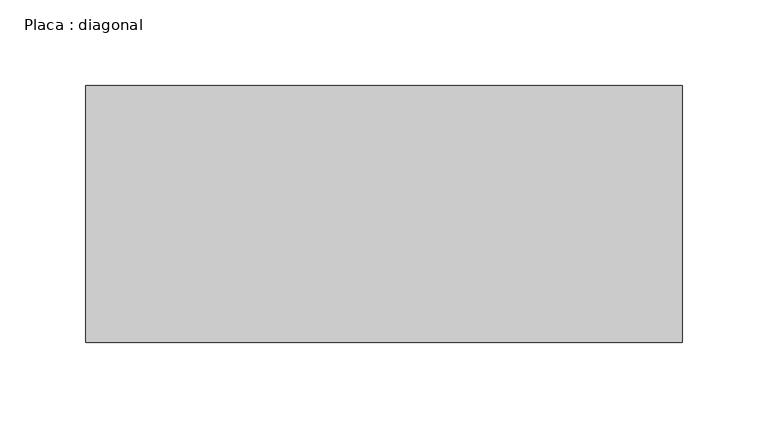
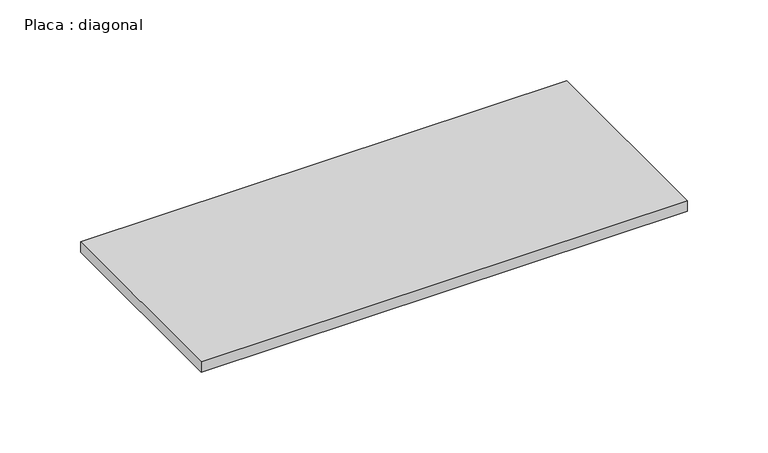
"""IFC4 building model written with IfcOpenShell, lengths in millimetres: beam geometry, Placa : diagonal."""

import ifcopenshell
import ifcopenshell.guid

model = None  # the IFC model being written
_history = None  # IfcOwnerHistory: only IFC2X3 demands one
_inside = {}  # id of a spatial element -> (the spatial element, [elements in it])
_under = {}  # id of a project, library or spatial element -> (it, [spatial elements below it])
_declared = {}  # id of a project -> (the project, [libraries it declares])
_typed = {}  # id of a type object -> (the type object, [elements of that type])
_made_of = {}  # id of a material, layer set ... -> (it, [elements and type objects made of it])


def new_model(schema):
    """Start an empty IFC model of exactly this schema.

    Asked for "IFC4X3", IfcOpenShell would pick the latest addendum, in which some entities
    have other attributes; the version numbers below select the first issue.
    IFC2X3 requires an IfcOwnerHistory on every rooted entity: one is made here for all.
    """
    global model, _history
    if schema == "IFC4X3":
        model = ifcopenshell.file(schema_version=(4, 3, 0, 0))
    else:
        model = ifcopenshell.file(schema=schema)
    _inside.clear()
    _under.clear()
    _declared.clear()
    _typed.clear()
    _made_of.clear()
    _history = None
    if model.schema == "IFC2X3":
        org = make("IfcOrganization", Name="unknown")
        user = make(
            "IfcPersonAndOrganization",
            ThePerson=make("IfcPerson", FamilyName="unknown"),
            TheOrganization=org,
        )
        app = make(
            "IfcApplication",
            ApplicationDeveloper=org,
            Version="unknown",
            ApplicationFullName="unknown",
            ApplicationIdentifier="unknown",
        )
        _history = make(
            "IfcOwnerHistory",
            OwningUser=user,
            OwningApplication=app,
            ChangeAction="ADDED",
            CreationDate=0,
        )
    return model


def make(cls, **values):
    """One entity of the class cls with the attributes given. An attribute that is None is left unset."""
    return model.create_entity(
        cls, **{name: value for name, value in values.items() if value is not None}
    )


def rooted(cls, **values):
    """An entity with a GlobalId (a new one), such as an element, a storey or a relation."""
    return make(cls, GlobalId=ifcopenshell.guid.new(), OwnerHistory=_history, **values)


def si_unit(unit_type, name, prefix=None):
    """IfcSIUnit, for example si_unit("LENGTHUNIT", "METRE", prefix="MILLI")."""
    return make("IfcSIUnit", UnitType=unit_type, Prefix=prefix, Name=name)


def assignment(units):
    """IfcUnitAssignment: the units of a project."""
    return None if units is None else make("IfcUnitAssignment", Units=units)


def point(xyz):
    """IfcCartesianPoint."""
    return None if xyz is None else make("IfcCartesianPoint", Coordinates=xyz)


def direction(xyz):
    """IfcDirection."""
    return None if xyz is None else make("IfcDirection", DirectionRatios=xyz)


def frame(location, z_axis=None, x_axis=None):
    """IfcAxis2Placement3D, a coordinate frame: its origin and axes. An axis left out is left unset."""
    return make(
        "IfcAxis2Placement3D",
        Location=point(location),
        Axis=direction(z_axis),
        RefDirection=direction(x_axis),
    )


def origin():
    """The frame at (0, 0, 0) with its axes left unset."""
    return frame((0.0, 0.0, 0.0))


def place(relative_to, where):
    """IfcLocalPlacement: puts the frame where relative to a parent placement (None: the world)."""
    return make(
        "IfcLocalPlacement", PlacementRelTo=relative_to, RelativePlacement=where
    )


def context(
    kind, dimensions, precision=None, world=None, true_north=None, identifier=None
):
    """IfcGeometricRepresentationContext, for example the 3D "Model" context."""
    return make(
        "IfcGeometricRepresentationContext",
        ContextIdentifier=identifier,
        ContextType=kind,
        CoordinateSpaceDimension=dimensions,
        Precision=precision,
        WorldCoordinateSystem=world,
        TrueNorth=true_north,
    )


def project(units=None, contexts=None):
    """IfcProject with its units and contexts."""
    return rooted(
        "IfcProject",
        Name="project",
        RepresentationContexts=contexts,
        UnitsInContext=assignment(units),
    )


def spatial(cls, under=None, at=None, **own):
    """A site, building, storey or space (cls), placed at a placement, below another one or the project."""
    s = rooted(cls, ObjectPlacement=at, **own)
    if under is not None:
        _under.setdefault(under.id(), (under, []))[1].append(s)
    return s


def polyline(points):
    """IfcPolyline through the points."""
    return make("IfcPolyline", Points=[point(p) for p in points])


def outline(outer, holes=None, kind="AREA"):
    """IfcArbitraryClosedProfileDef: a profile drawn as a closed curve; with holes, ...WithVoids."""
    if holes is None:
        return make("IfcArbitraryClosedProfileDef", ProfileType=kind, OuterCurve=outer)
    return make(
        "IfcArbitraryProfileDefWithVoids",
        ProfileType=kind,
        OuterCurve=outer,
        InnerCurves=holes,
    )


def extrude(swept, where, along, depth):
    """IfcExtrudedAreaSolid: the profile swept, set in the frame where, extruded along a direction by depth."""
    return make(
        "IfcExtrudedAreaSolid",
        SweptArea=swept,
        Position=where,
        ExtrudedDirection=direction(along),
        Depth=depth,
    )


def shape(context_of_items, identifier, shape_type, items):
    """IfcShapeRepresentation: the items that make up one representation, for example the "Body"."""
    return make(
        "IfcShapeRepresentation",
        ContextOfItems=context_of_items,
        RepresentationIdentifier=identifier,
        RepresentationType=shape_type,
        Items=items,
    )


def source(mapping_origin, context_of_items, identifier, shape_type, items):
    """IfcRepresentationMap: a shape defined once, which mapped items show again and again."""
    return make(
        "IfcRepresentationMap",
        MappingOrigin=mapping_origin,
        MappedRepresentation=shape(context_of_items, identifier, shape_type, items),
    )


def transform(
    local_origin,
    x_axis=None,
    y_axis=None,
    z_axis=None,
    scale=None,
    scale2=None,
    scale3=None,
    uniform=True,
):
    """IfcCartesianTransformationOperator3D, or its non-uniform kind. x_axis, y_axis, z_axis: its Axis1, 2, 3."""
    if uniform:
        return make(
            "IfcCartesianTransformationOperator3D",
            Axis1=direction(x_axis),
            Axis2=direction(y_axis),
            LocalOrigin=point(local_origin),
            Scale=scale,
            Axis3=direction(z_axis),
        )
    return make(
        "IfcCartesianTransformationOperator3DnonUniform",
        Axis1=direction(x_axis),
        Axis2=direction(y_axis),
        LocalOrigin=point(local_origin),
        Scale=scale,
        Axis3=direction(z_axis),
        Scale2=scale2,
        Scale3=scale3,
    )


def mapped(mapping_source, mapping_target):
    """IfcMappedItem: shows the shape of a source again, moved by a transform."""
    return make(
        "IfcMappedItem", MappingSource=mapping_source, MappingTarget=mapping_target
    )


def made_of(thing, what):
    """Note that an element or type object is made of a material, layer set ...; save() writes the relation."""
    if what is not None:
        _made_of.setdefault(what.id(), (what, []))[1].append(thing)
    return thing


def element(
    cls,
    number,
    at=None,
    inside=None,
    cuts=None,
    type_object=None,
    material=None,
    context=None,
    identifier="Body",
    shape_type=None,
    held_by="IfcProductDefinitionShape",
    body=None,
    shapes=None,
    **own,
):
    """One element of the class cls, such as IfcWall. Its Tag is "e" and its number.

    at: its placement. inside: the storey or other place that contains it. cuts: it is an
    opening in that element (IfcRelVoidsElement). A single representation is given by context,
    identifier, shape_type and body (its items); several are given by shapes. held_by: the class
    of the entity that holds the representations. save() writes the other relations.
    """
    e = rooted(cls, Tag="e%d" % number, ObjectPlacement=at, **own)
    if body is not None:
        shapes = [shape(context, identifier, shape_type, body)]
    if shapes is not None:
        e.Representation = make(held_by, Representations=shapes)
    if inside is not None:
        _inside.setdefault(inside.id(), (inside, []))[1].append(e)
    if cuts is not None:
        rooted(
            "IfcRelVoidsElement", RelatingBuildingElement=cuts, RelatedOpeningElement=e
        )
    if type_object is not None:
        _typed.setdefault(type_object.id(), (type_object, []))[1].append(e)
    return made_of(e, material)


def aggregate(whole, parts):
    """IfcRelAggregates: a whole, such as a stair, and the parts it consists of."""
    return rooted("IfcRelAggregates", RelatingObject=whole, RelatedObjects=parts)


def save(model, path):
    """Write the relations noted so far, then the file.

    IfcRelAggregates (storeys below a building ...), IfcRelContainedInSpatialStructure (elements
    in a storey), IfcRelDefinesByType, IfcRelAssociatesMaterial and IfcRelDeclares: one each for
    every whole, place, type object, material and project.
    """
    for whole, parts in _under.values():
        aggregate(whole, parts)
    for where, things in _inside.values():
        rooted(
            "IfcRelContainedInSpatialStructure",
            RelatedElements=things,
            RelatingStructure=where,
        )
    for kind, things in _typed.values():
        rooted("IfcRelDefinesByType", RelatedObjects=things, RelatingType=kind)
    for what, things in _made_of.values():
        rooted("IfcRelAssociatesMaterial", RelatedObjects=things, RelatingMaterial=what)
    for by, libraries in _declared.values():
        rooted("IfcRelDeclares", RelatingContext=by, RelatedDefinitions=libraries)
    model.write(path)


def placa_diagonal_cdd87bdc(model_context):
    return source(origin(), model_context, "Body", "SweptSolid", [
        extrude(outline(polyline([(162.1535761, 75.0), (162.1535761, -75.0), (-186.2011239, -75.0), (-186.2011239, 75.0), (162.1535761, 75.0)])), frame((0.0, 0.0, -4.0), z_axis=(0.0, 0.0, 1.0), x_axis=(1.0, 0.0, 0.0)), (0.0, 0.0, 1.0), 8.0),
    ])


if __name__ == "__main__":
    model = new_model("IFC4")
    model_context = context("Model", 3, world=origin())
    ifc_project = project(units=[si_unit("LENGTHUNIT", "METRE", prefix="MILLI")], contexts=[model_context])
    site = spatial("IfcSite", under=ifc_project)
    building = spatial("IfcBuilding", under=site)
    placement = place(None, origin())
    placa_diagonal_shape = placa_diagonal_cdd87bdc(model_context)
    element("IfcBeam", 1, ObjectType="Placa : diagonal", at=placement, inside=building, context=model_context, shape_type="MappedRepresentation", body=[
        mapped(placa_diagonal_shape, transform((0.0, 0.0, 0.0), x_axis=(1.0, 0.0, 0.0), y_axis=(0.0, 1.0, 0.0), z_axis=(0.0, 0.0, 1.0))),
    ])
    save(model, "model.ifc")

# Revit data of these elements
# Type "Placa : diagonal"
#   W = 0
#   Length [instance default] = 1.50 m
#   b = 0.15 m
#   d = 0.008 m
#   A = 0 m²
#   Structural Material [instance default] = Aço, 45-345
# Element 1 (IfcBeam, "Placa : diagonal")
#   Materials on its faces: "Aço, 45-345"
# Materials
#   "Aço, 45-345": class "Metal", colour RGB 247 247 247, transparency 0, Description = "Aço 345 MPa", Cost = 0
